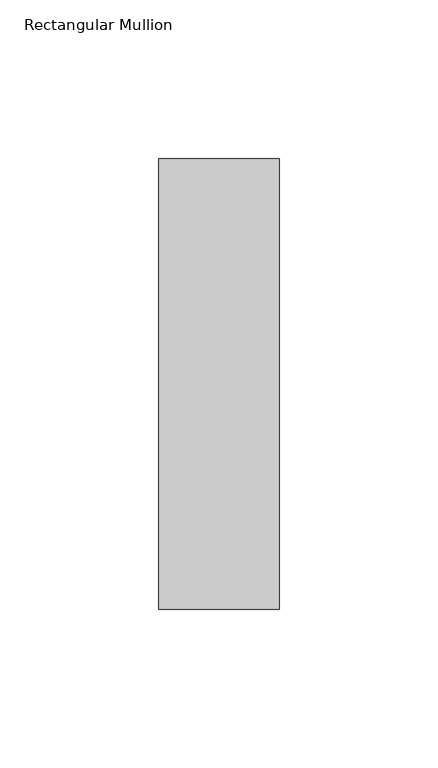
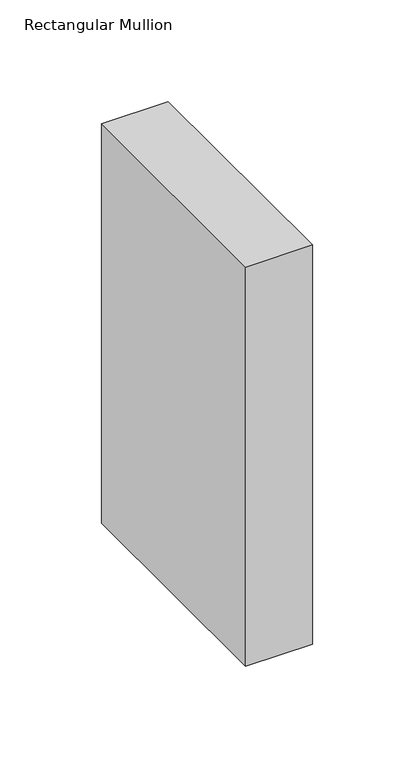
"""IFC4 building model written with IfcOpenShell, lengths in millimetres: member geometry, Rectangular Mullion : NLRS_21_CWM_hsb-regel 38x142_gen_rsf."""

from ifc_helpers import new_model, si_unit, frame, origin, place, context, project, spatial, polyline, outline, extrude, source, transform, mapped, element, save


def rectangular_mullion_ad7c5b17(model_context):
    return source(origin(), model_context, "Body", "SweptSolid", [
        extrude(outline(polyline([(-38.0, -71.0), (-38.0, 71.0), (0.0, 71.0), (0.0, -71.0), (-38.0, -71.0)])), frame((0.0, 0.0, -239.8441061), z_axis=(0.0, 0.0, 1.0), x_axis=(1.0, 0.0, 0.0)), (0.0, 0.0, 1.0), 239.8441061),
    ])


if __name__ == "__main__":
    model = new_model("IFC4")
    model_context = context("Model", 3, world=origin())
    ifc_project = project(units=[si_unit("LENGTHUNIT", "METRE", prefix="MILLI")], contexts=[model_context])
    site = spatial("IfcSite", under=ifc_project)
    building = spatial("IfcBuilding", under=site)
    placement = place(None, origin())
    rectangular_mullion_shape = rectangular_mullion_ad7c5b17(model_context)
    element("IfcMember", 1, ObjectType="Rectangular Mullion : NLRS_21_CWM_hsb-regel 38x142_gen_rsf", at=placement, inside=building, context=model_context, shape_type="MappedRepresentation", body=[
        mapped(rectangular_mullion_shape, transform((0.0, 0.0, 0.0), x_axis=(1.0, 0.0, 0.0), y_axis=(0.0, 1.0, 0.0), z_axis=(0.0, 0.0, 1.0))),
    ])
    save(model, "model.ifc")

# Revit data of these elements
# Type "Rectangular Mullion : NLRS_21_CWM_hsb-regel 38x142_gen_rsf"
#   Export Type to IFC As = "IfcWall"
#   Type IfcGUID = "07M7mRoiH1CR8m_RSKIwpF"
#   Assembly Code = "21.10"
#   built-in parameter 1007322 = 0.465879 (stored number, unit not read)
#   built-in parameter 1007321 = 0.062336 (stored number, unit not read)
#   built-in parameter 1007320 = 0.062336 (stored number, unit not read)
# Element 1 (IfcMember, "Rectangular Mullion : NLRS_21_CWM_hsb-regel 38x142_gen_rsf")
#   Materials on its faces: "NLRS_i2_hout naaldhout vuren_gen_rsf"
# Materials
#   "NLRS_i2_hout naaldhout vuren_gen_rsf": class "I - Hout", colour RGB 234 199 147, transparency 0, Keynote = "i2", Manufacturer = "Revit Standards Foundation", URL = "www.revitstandards.org", Description = "hout vuren", Cost = 0
